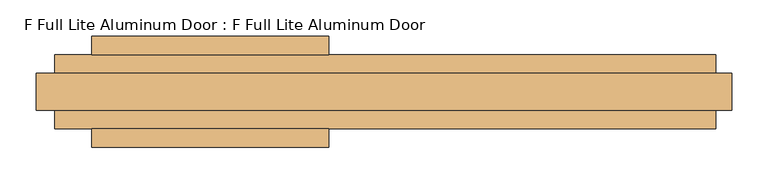
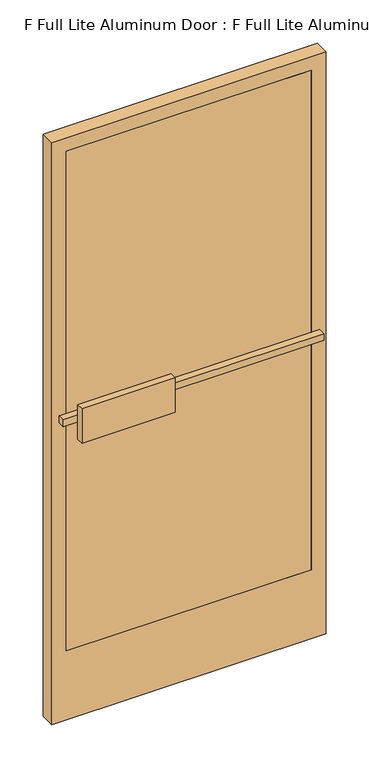
"""IFC4 building model written with IfcOpenShell, lengths in millimetres: door geometry, F Full Lite Aluminum Door : F Full Lite Aluminum Door."""

from ifc_helpers import new_model, si_unit, frame, origin, place, context, project, spatial, polyline, outline, extrude, source, transform, mapped, element, save


def f_full_lite_aluminum_door_f_full_lite_aluminum_door_618387bc(model_context):
    return source(origin(), model_context, "Body", "SweptSolid", [
        extrude(outline(polyline([(427.434375, 0.0), (-427.434375, 0.0), (-427.434375, 50.8), (427.434375, 50.8), (427.434375, 0.0)])), frame((0.0, 0.0, 254.0), z_axis=(0.0, 0.0, 1.0), x_axis=(1.0, 0.0, 0.0)), (0.0, 0.0, 1.0), 1840.70625),
        extrude(outline(polyline([(2145.50625, -478.234375), (0.0, -478.234375), (0.0, 478.234375), (2145.50625, 478.234375), (2145.50625, -478.234375)]), holes=[polyline([(2094.70625, -427.434375), (2094.70625, 427.434375), (254.0, 427.434375), (254.0, -427.434375), (2094.70625, -427.434375)])]), frame((0.0, 0.0, 0.0), z_axis=(0.0, 1.0, 0.0), x_axis=(0.0, 0.0, 1.0)), (0.0, 0.0, 1.0), 50.8),
        extrude(outline(polyline([(-402.034375, -25.4), (-76.2, -25.4), (-76.2, -50.8), (-402.034375, -50.8), (-402.034375, -25.4)])), frame((0.0, 0.0, 1041.4), z_axis=(0.0, 0.0, 1.0), x_axis=(1.0, 0.0, 0.0)), (0.0, 0.0, 1.0), 127.0),
        extrude(outline(polyline([(-76.2, 76.2), (-402.034375, 76.2), (-402.034375, 101.6), (-76.2, 101.6), (-76.2, 76.2)])), frame((0.0, 0.0, 1053.30625), z_axis=(0.0, 0.0, 1.0), x_axis=(1.0, 0.0, 0.0)), (0.0, 0.0, 1.0), 127.0),
        extrude(outline(polyline([(-452.834375, 0.0), (456.4629464, 0.0), (456.4629464, -25.4), (-452.834375, -25.4), (-452.834375, 0.0)])), frame((0.0, 0.0, 1104.10625), z_axis=(0.0, 0.0, 1.0), x_axis=(1.0, 0.0, 0.0)), (0.0, 0.0, 1.0), 25.4),
        extrude(outline(polyline([(456.4629464, 50.8), (-452.834375, 50.8), (-452.834375, 76.2), (456.4629464, 76.2), (456.4629464, 50.8)])), frame((0.0, 0.0, 1092.2), z_axis=(0.0, 0.0, 1.0), x_axis=(1.0, 0.0, 0.0)), (0.0, 0.0, 1.0), 25.4),
    ])


if __name__ == "__main__":
    model = new_model("IFC4")
    model_context = context("Model", 3, world=origin())
    ifc_project = project(units=[si_unit("LENGTHUNIT", "METRE", prefix="MILLI")], contexts=[model_context])
    site = spatial("IfcSite", under=ifc_project)
    building = spatial("IfcBuilding", under=site)
    placement = place(None, origin())
    f_full_lite_aluminum_door_f_full_lite_aluminum_door_shape = f_full_lite_aluminum_door_f_full_lite_aluminum_door_618387bc(model_context)
    element("IfcDoor", 1, ObjectType="F Full Lite Aluminum Door : F Full Lite Aluminum Door", at=placement, inside=building, context=model_context, shape_type="MappedRepresentation", body=[
        mapped(f_full_lite_aluminum_door_f_full_lite_aluminum_door_shape, transform((0.0, 0.0, 0.0), x_axis=(1.0, 0.0, 0.0), y_axis=(0.0, 1.0, 0.0), z_axis=(0.0, 0.0, 1.0))),
    ])
    save(model, "model.ifc")

# Revit data of these elements
# Type "F Full Lite Aluminum Door : F Full Lite Aluminum Door"
#   Type Mark = "20"
#   Construction Type Id = "SGL"
#   Assembly Code = "B2030100"
#   Analytic Construction = "Large single-glazed windows"
#   Visual Light Transmittance = 0.9
#   Thermal Resistance (R) = 0.179801 (m²·K)/W
#   Solar Heat Gain Coefficient = 0.86
#   Heat Transfer Coefficient (U) = 5.5617 W/(m²·K)
#   Offset = 0' - 2"
#   Function = 1
#   Handle Material = Aluminum
#   Glazing Material = Glass
# Element 1 (IfcDoor, "F Full Lite Aluminum Door : F Full Lite Aluminum Door")
#   Materials on its faces: "Aluminum", "Glass"
# Materials
#   "Aluminum": class "Metal", colour RGB 247 247 247, transparency 0, Description = "Aluminum 6061", Cost = 0
#   "Glass": class "Unassigned", colour RGB 0 0 255, transparency 0.75
